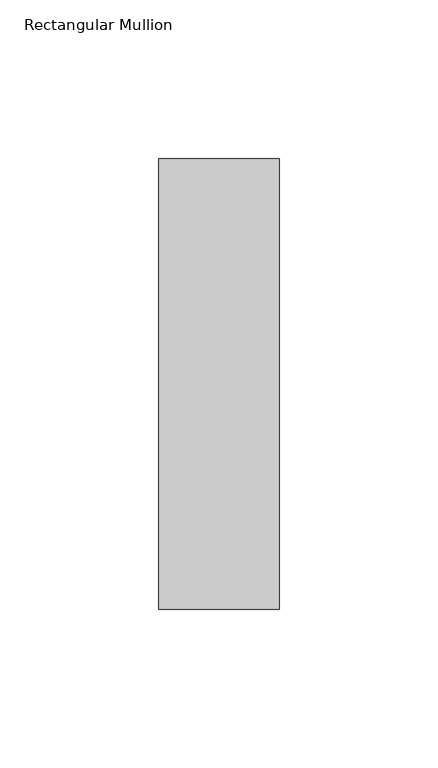
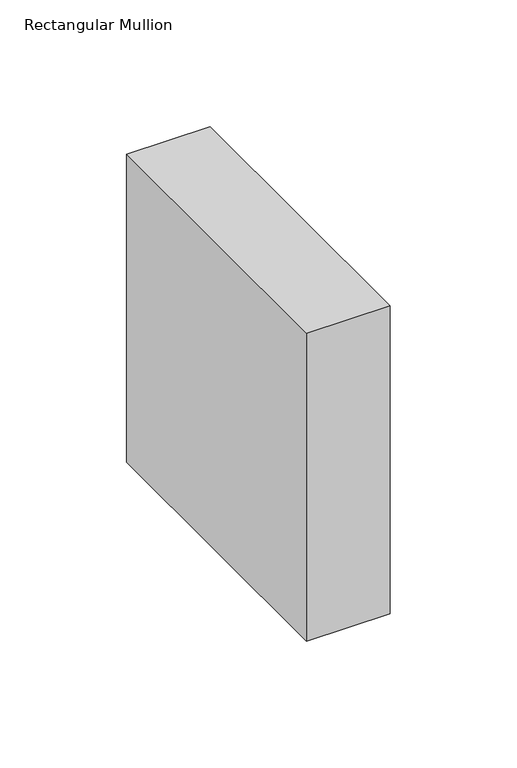
"""IFC4 building model written with IfcOpenShell, lengths in millimetres: member geometry, Rectangular Mullion : NLRS_21_CWM_hsb-regel 38x142_gen_rsf."""

from ifc_helpers import new_model, si_unit, frame, origin, place, context, project, spatial, polyline, outline, extrude, source, transform, mapped, element, save


def rectangular_mullion_8a963fb8(model_context):
    return source(origin(), model_context, "Body", "SweptSolid", [
        extrude(outline(polyline([(19.0, -71.0), (-19.0, -71.0), (-19.0, 71.0), (19.0, 71.0), (19.0, -71.0)])), frame((0.0, 0.0, -148.1558939), z_axis=(0.0, 0.0, 1.0), x_axis=(1.0, 0.0, 0.0)), (0.0, 0.0, 1.0), 148.1558939),
    ])


if __name__ == "__main__":
    model = new_model("IFC4")
    model_context = context("Model", 3, world=origin())
    ifc_project = project(units=[si_unit("LENGTHUNIT", "METRE", prefix="MILLI")], contexts=[model_context])
    site = spatial("IfcSite", under=ifc_project)
    building = spatial("IfcBuilding", under=site)
    placement = place(None, origin())
    rectangular_mullion_shape = rectangular_mullion_8a963fb8(model_context)
    element("IfcMember", 1, ObjectType="Rectangular Mullion : NLRS_21_CWM_hsb-regel 38x142_gen_rsf", at=placement, inside=building, context=model_context, shape_type="MappedRepresentation", body=[
        mapped(rectangular_mullion_shape, transform((0.0, 0.0, 0.0), x_axis=(1.0, 0.0, 0.0), y_axis=(0.0, 1.0, 0.0), z_axis=(0.0, 0.0, 1.0))),
    ])
    save(model, "model.ifc")

# Revit data of these elements
# Type "Rectangular Mullion : NLRS_21_CWM_hsb-regel 38x142_gen_rsf"
#   Export Type to IFC As = "IfcWall"
#   Type IfcGUID = "07M7mRoiH1CR8m_RSKIwpF"
#   Assembly Code = "21.10"
#   built-in parameter 1007322 = 0.465879 (stored number, unit not read)
#   built-in parameter 1007321 = 0.062336 (stored number, unit not read)
#   built-in parameter 1007320 = 0.062336 (stored number, unit not read)
# Element 1 (IfcMember, "Rectangular Mullion : NLRS_21_CWM_hsb-regel 38x142_gen_rsf")
#   Materials on its faces: "NLRS_i2_hout naaldhout vuren_gen_rsf"
# Materials
#   "NLRS_i2_hout naaldhout vuren_gen_rsf": class "I - Hout", colour RGB 234 199 147, transparency 0, Keynote = "i2", Manufacturer = "Revit Standards Foundation", URL = "www.revitstandards.org", Description = "hout vuren", Cost = 0
